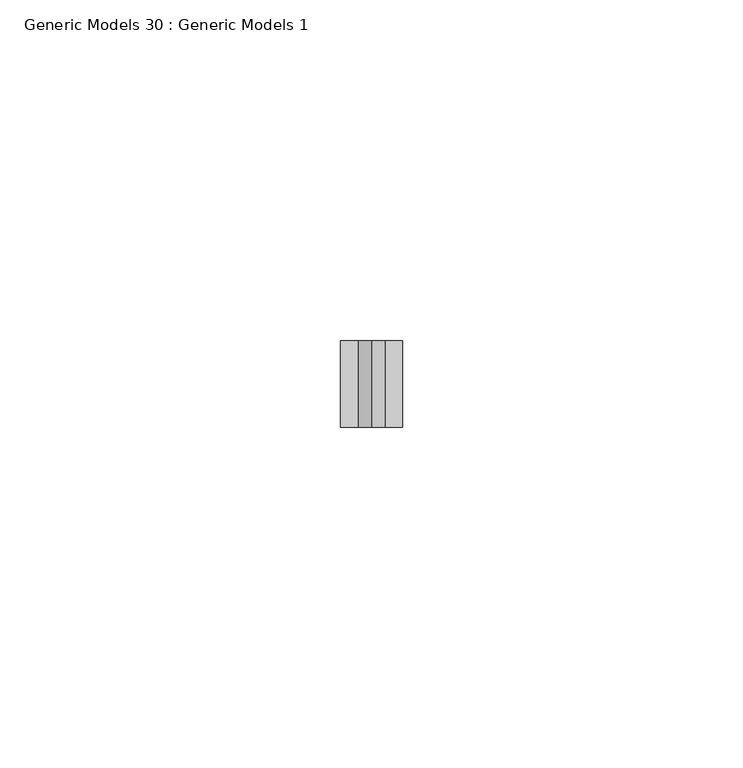
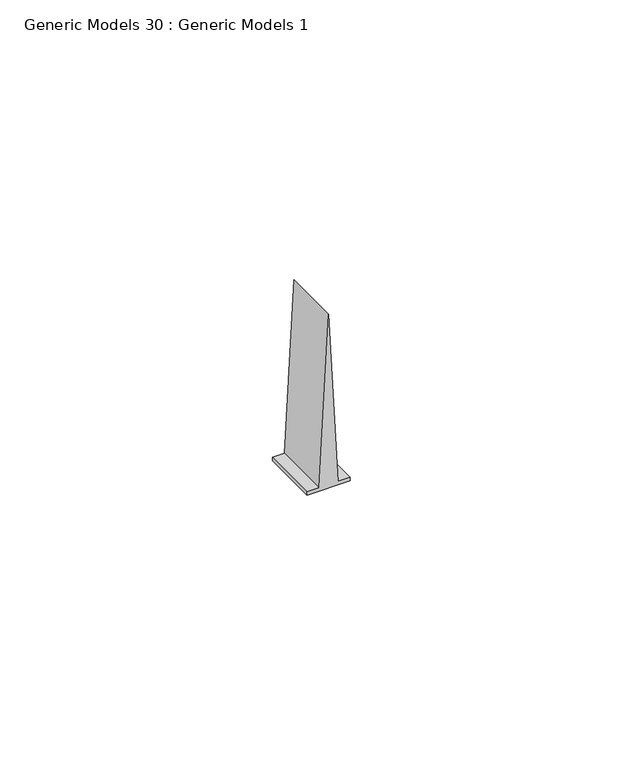
"""IFC4 building model written with IfcOpenShell, lengths in millimetres: proxy geometry, Generic Models 30 : Generic Models 1."""

from ifc_helpers import new_model, si_unit, frame, origin, place, context, project, spatial, polyline, outline, extrude, source, transform, mapped, element, save


def generic_models_30_generic_models_1_77c62db4(model_context):
    return source(origin(), model_context, "Body", "SweptSolid", [
        extrude(outline(polyline([(2429.7615469, 49845.474547), (2429.7615469, 49854.567747), (2430.5552969, 49854.567747), (2430.5552969, 49852.0178834), (2468.6552969, 49850.021147), (2430.5552969, 49848.0244106), (2430.5552969, 49845.474547), (2429.7615469, 49845.474547)])), frame((0.0, 565.15, 0.0), z_axis=(0.0, 1.0, 0.0), x_axis=(0.0, 0.0, 1.0)), (0.0, 0.0, 1.0), 12.7),
    ])


if __name__ == "__main__":
    model = new_model("IFC4")
    model_context = context("Model", 3, world=origin())
    ifc_project = project(units=[si_unit("LENGTHUNIT", "METRE", prefix="MILLI")], contexts=[model_context])
    site = spatial("IfcSite", under=ifc_project)
    building = spatial("IfcBuilding", under=site)
    placement = place(None, origin())
    generic_models_30_generic_models_1_shape = generic_models_30_generic_models_1_77c62db4(model_context)
    element("IfcBuildingElementProxy", 1, Name="Generic Models 30 : Generic Models 1", ObjectType="Generic Models 30 : Generic Models 1", at=placement, inside=building, context=model_context, shape_type="MappedRepresentation", body=[
        mapped(generic_models_30_generic_models_1_shape, transform((0.0, 0.0, 0.0), x_axis=(1.0, 0.0, 0.0), y_axis=(0.0, 1.0, 0.0), z_axis=(0.0, 0.0, 1.0))),
    ])
    save(model, "model.ifc")

# Revit data of these elements
# Element 1 (IfcBuildingElementProxy, "Generic Models 30 : Generic Models 1")
#   Materials on its faces: "ATTACH GYPSUM BOARD TO STUDS AND NOT TO TOP TRACK"
# Materials
#   "ATTACH GYPSUM BOARD TO STUDS AND NOT TO TOP TRACK": class "Generic", colour RGB 48 48 48, transparency 0, Cost = 0
